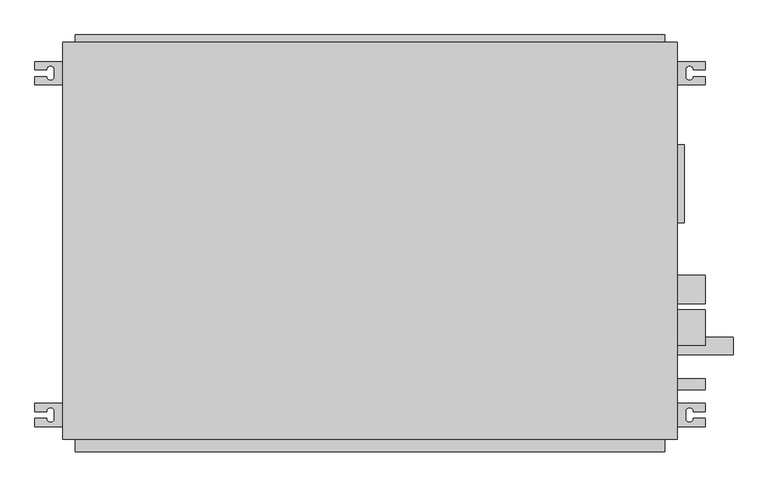
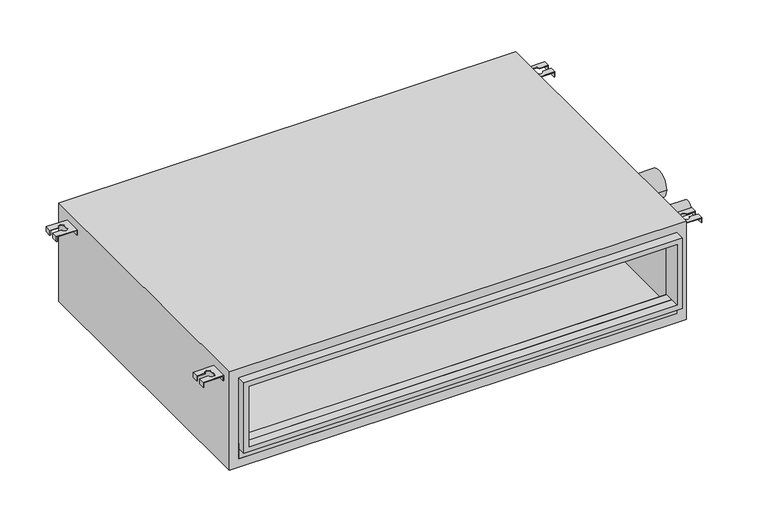
"""IFC4 building model written with IfcOpenShell, lengths in millimetres: proxy geometry, PEFY-P-NMAU-E_Medium_Static_Ducted : PEFY-P30NMAU-E."""

from ifc_helpers import new_model, si_unit, point, frame, frame_2d, origin, place, context, project, spatial, polyline, circle_curve, trimmed, segment, composite_curve, outline, extrude, source, transform, mapped, element, save
from ifc_brep_helpers import plane_surface, revolved_surface, advanced_brep


def mechanical_equipment_d42a0ae8(model_context):
    return source(origin(), model_context, "Body", "SolidModel", [
        advanced_brep(
        [(-610.087243, -231.05, 249.2375), (-610.087243, -246.05, 249.2375), (-589.080993, -246.05, 249.2375), (-575.080993, -246.05, 249.2375), (-575.080993, -258.05, 249.2375), (-589.080993, -258.05, 249.2375), (-610.087243, -258.05, 249.2375), (-610.087243, -273.05, 249.2375), (-560.080993, -273.05, 249.2375), (-560.080993, -231.05, 249.2375), (-610.087243, -231.05, 236.4972162), (-608.499243, -231.05, 236.4972162), (-608.499243, -246.05, 236.4972162), (-610.087243, -246.05, 236.4972162), (-608.499243, -273.05, 236.4972162), (-610.087243, -273.05, 236.4972162), (-610.087243, -258.05, 236.4972162), (-608.499243, -258.05, 236.4972162), (-560.080993, -231.05, 236.4972162), (-560.080993, -273.05, 236.4972162), (-561.668993, -273.05, 236.4972162), (-561.668993, -231.05, 236.4972162), (-608.499243, -246.05, 247.65), (-589.080993, -246.05, 247.65), (-608.499243, -231.05, 247.65), (-561.668993, -231.05, 247.65), (-608.499243, -258.05, 247.65), (-608.499243, -273.05, 247.65), (-589.080993, -258.05, 247.65), (-561.668993, -273.05, 247.65), (-575.080993, -258.05, 247.65), (-575.080993, -246.05, 247.65)],
        [
            (0, 1),
            (1, 2),
            (2, 3, circle_curve(frame((-582.080993, -246.05, 249.2375), z_axis=(0.0, 0.0, -1.0), x_axis=(1.0, 0.0, 0.0)), 7.0)),
            (3, 4),
            (4, 5, circle_curve(frame((-582.080993, -258.05, 249.2375), z_axis=(0.0, 0.0, -1.0), x_axis=(1.0, 0.0, 0.0)), 7.0)),
            (5, 6),
            (6, 7),
            (7, 8),
            (8, 9),
            (9, 0),
            (10, 11),
            (11, 12),
            (12, 13),
            (13, 10),
            (14, 15),
            (15, 16),
            (16, 17),
            (17, 14),
            (18, 19),
            (19, 20),
            (20, 21),
            (21, 18),
            (13, 1),
            (0, 10),
            (12, 22),
            (22, 23),
            (23, 2),
            (11, 24),
            (24, 22),
            (9, 18),
            (21, 25),
            (25, 24),
            (17, 26),
            (26, 27),
            (27, 14),
            (5, 28),
            (28, 26),
            (16, 6),
            (15, 7),
            (27, 29),
            (29, 20),
            (19, 8),
            (29, 25),
            (30, 31),
            (31, 23, circle_curve(frame((-582.080993, -246.05, 247.65), z_axis=(0.0, 0.0, 1.0), x_axis=(1.0, 0.0, 0.0)), 7.0)),
            (28, 30, circle_curve(frame((-582.080993, -258.05, 247.65), z_axis=(0.0, 0.0, 1.0), x_axis=(1.0, 0.0, 0.0)), 7.0)),
            (4, 30),
            (31, 3),
        ],
        [
            plane_surface(frame((-610.087243, -231.05, 249.2375), z_axis=(0.0, 0.0, 1.0), x_axis=(0.0, -1.0, 0.0))),
            plane_surface(frame((-610.087243, -231.05, 236.4972162), z_axis=(0.0, 0.0, -1.0), x_axis=(0.0, 1.0, 0.0))),
            plane_surface(frame((-610.087243, -231.05, 249.2375), z_axis=(-1.0, 0.0, 0.0), x_axis=(0.0, 0.0, -1.0))),
            plane_surface(frame((-610.087243, -246.05, 249.2375), z_axis=(0.0, -1.0, 0.0), x_axis=(0.0, 0.0, -1.0))),
            plane_surface(frame((-608.499243, -246.05, 249.2375), z_axis=(1.0, 0.0, 0.0), x_axis=(0.0, 0.0, -1.0))),
            plane_surface(frame((-608.499243, -231.05, 249.2375), z_axis=(0.0, 1.0, 0.0), x_axis=(0.0, 0.0, -1.0))),
            plane_surface(frame((-608.499243, -273.05, 249.2375), z_axis=(1.0, 0.0, 0.0), x_axis=(0.0, 0.0, -1.0))),
            plane_surface(frame((-608.499243, -258.05, 249.2375), z_axis=(0.0, 1.0, 0.0), x_axis=(0.0, 0.0, -1.0))),
            plane_surface(frame((-610.087243, -258.05, 249.2375), z_axis=(-1.0, 0.0, 0.0), x_axis=(0.0, 0.0, -1.0))),
            plane_surface(frame((-610.087243, -273.05, 249.2375), z_axis=(0.0, -1.0, 0.0), x_axis=(0.0, 0.0, -1.0))),
            plane_surface(frame((-561.668993, -231.05, 249.2375), z_axis=(-1.0, 0.0, 0.0), x_axis=(0.0, 0.0, -1.0))),
            plane_surface(frame((-560.080993, -273.05, 249.2375), z_axis=(1.0, 0.0, 0.0), x_axis=(0.0, 0.0, -1.0))),
            plane_surface(frame((-575.080993, -258.05, 247.65), z_axis=(0.0, 0.0, -1.0), x_axis=(0.0, 1.0, 0.0))),
            revolved_surface(polyline([(-575.080993, -258.05, 247.65), (-575.080993, -258.05, 249.2375)]), (-582.080993, -258.05, 247.65), (0.0, 0.0, -1.0)),
            revolved_surface(polyline([(-575.080993, -246.05, 247.65), (-575.080993, -246.05, 249.2375)]), (-582.080993, -246.05, 247.65), (0.0, 0.0, -1.0)),
            plane_surface(frame((-575.080993, -246.05, 249.2375), z_axis=(-1.0, 0.0, 0.0), x_axis=(0.0, 0.0, -1.0))),
        ],
        [
            (0, [[1, 2, 3, 4, 5, 6, 7, 8, 9, 10]]),
            (1, [[11, 12, 13, 14]]),
            (1, [[15, 16, 17, 18]]),
            (1, [[19, 20, 21, 22]]),
            (2, [[23, -1, 24, -14]]),
            (3, [[-2, -23, -13, 25, 26, 27]]),
            (4, [[-12, 28, 29, -25]]),
            (5, [[-10, 30, -22, 31, 32, -28, -11, -24]]),
            (6, [[-18, 33, 34, 35]]),
            (7, [[-6, 36, 37, -33, -17, 38]]),
            (8, [[39, -7, -38, -16]]),
            (9, [[-8, -39, -15, -35, 40, 41, -20, 42]]),
            (10, [[-21, -41, 43, -31]]),
            (11, [[-30, -9, -42, -19]]),
            (12, [[44, 45, -26, -29, -32, -43, -40, -34, -37, 46]]),
            (13, [[-5, 47, -46, -36]]),
            (14, [[-3, -27, -45, 48]]),
            (15, [[-4, -48, -44, -47]]),
        ],
    ),
        advanced_brep(
        [(590.062757, -231.05, 249.2375), (540.056507, -231.05, 249.2375), (540.056507, -273.05, 249.2375), (590.062757, -273.05, 249.2375), (590.062757, -258.05, 249.2375), (569.056507, -258.05, 249.2375), (555.056507, -258.05, 249.2375), (555.056507, -246.05, 249.2375), (569.056507, -246.05, 249.2375), (590.062757, -246.05, 249.2375), (590.062757, -231.05, 236.4972162), (590.062757, -246.05, 236.4972162), (588.474757, -246.05, 236.4972162), (588.474757, -231.05, 236.4972162), (588.474757, -273.05, 236.4972162), (588.474757, -258.05, 236.4972162), (590.062757, -258.05, 236.4972162), (590.062757, -273.05, 236.4972162), (540.056507, -231.05, 236.4972162), (541.644507, -231.05, 236.4972162), (541.644507, -273.05, 236.4972162), (540.056507, -273.05, 236.4972162), (569.056507, -246.05, 247.65), (588.474757, -246.05, 247.65), (588.474757, -231.05, 247.65), (541.644507, -231.05, 247.65), (588.474757, -273.05, 247.65), (588.474757, -258.05, 247.65), (569.056507, -258.05, 247.65), (541.644507, -273.05, 247.65), (555.056507, -258.05, 247.65), (555.056507, -246.05, 247.65)],
        [
            (0, 1),
            (1, 2),
            (2, 3),
            (3, 4),
            (4, 5),
            (5, 6, circle_curve(frame((562.056507, -258.05, 249.2375), z_axis=(0.0, 0.0, -1.0), x_axis=(-1.0, 0.0, 0.0)), 7.0)),
            (6, 7),
            (7, 8, circle_curve(frame((562.056507, -246.05, 249.2375), z_axis=(0.0, 0.0, -1.0), x_axis=(-1.0, 0.0, 0.0)), 7.0)),
            (8, 9),
            (9, 0),
            (10, 11),
            (11, 12),
            (12, 13),
            (13, 10),
            (14, 15),
            (15, 16),
            (16, 17),
            (17, 14),
            (18, 19),
            (19, 20),
            (20, 21),
            (21, 18),
            (10, 0),
            (9, 11),
            (8, 22),
            (22, 23),
            (23, 12),
            (23, 24),
            (24, 13),
            (24, 25),
            (25, 19),
            (18, 1),
            (14, 26),
            (26, 27),
            (27, 15),
            (4, 16),
            (27, 28),
            (28, 5),
            (3, 17),
            (2, 21),
            (20, 29),
            (29, 26),
            (25, 29),
            (30, 28, circle_curve(frame((562.056507, -258.05, 247.65), z_axis=(0.0, 0.0, 1.0), x_axis=(-1.0, 0.0, 0.0)), 7.0)),
            (22, 31, circle_curve(frame((562.056507, -246.05, 247.65), z_axis=(0.0, 0.0, 1.0), x_axis=(-1.0, 0.0, 0.0)), 7.0)),
            (31, 30),
            (30, 6),
            (7, 31),
        ],
        [
            plane_surface(frame((590.062757, -231.05, 249.2375), z_axis=(0.0, 0.0, 1.0), x_axis=(0.0, -1.0, 0.0))),
            plane_surface(frame((590.062757, -231.05, 236.4972162), z_axis=(0.0, 0.0, -1.0), x_axis=(0.0, 1.0, 0.0))),
            plane_surface(frame((590.062757, -231.05, 249.2375), z_axis=(1.0, 0.0, 0.0), x_axis=(0.0, 0.0, -1.0))),
            plane_surface(frame((590.062757, -246.05, 249.2375), z_axis=(0.0, -1.0, 0.0), x_axis=(0.0, 0.0, -1.0))),
            plane_surface(frame((588.474757, -246.05, 249.2375), z_axis=(-1.0, 0.0, 0.0), x_axis=(0.0, 0.0, -1.0))),
            plane_surface(frame((588.474757, -231.05, 249.2375), z_axis=(0.0, 1.0, 0.0), x_axis=(0.0, 0.0, -1.0))),
            plane_surface(frame((588.474757, -273.05, 249.2375), z_axis=(-1.0, 0.0, 0.0), x_axis=(0.0, 0.0, -1.0))),
            plane_surface(frame((588.474757, -258.05, 249.2375), z_axis=(0.0, 1.0, 0.0), x_axis=(0.0, 0.0, -1.0))),
            plane_surface(frame((590.062757, -258.05, 249.2375), z_axis=(1.0, 0.0, 0.0), x_axis=(0.0, 0.0, -1.0))),
            plane_surface(frame((590.062757, -273.05, 249.2375), z_axis=(0.0, -1.0, 0.0), x_axis=(0.0, 0.0, -1.0))),
            plane_surface(frame((541.644507, -231.05, 249.2375), z_axis=(1.0, 0.0, 0.0), x_axis=(0.0, 0.0, -1.0))),
            plane_surface(frame((540.056507, -273.05, 249.2375), z_axis=(-1.0, 0.0, 0.0), x_axis=(0.0, 0.0, -1.0))),
            plane_surface(frame((555.056507, -258.05, 247.65), z_axis=(0.0, 0.0, -1.0), x_axis=(0.0, 1.0, 0.0))),
            revolved_surface(polyline([(555.056507, -258.05, 247.65), (555.056507, -258.05, 249.2375)]), (562.056507, -258.05, 247.65), (0.0, 0.0, -1.0)),
            revolved_surface(polyline([(555.056507, -246.05, 247.65), (555.056507, -246.05, 249.2375)]), (562.056507, -246.05, 247.65), (0.0, 0.0, -1.0)),
            plane_surface(frame((555.056507, -246.05, 249.2375), z_axis=(1.0, 0.0, 0.0), x_axis=(0.0, 0.0, -1.0))),
        ],
        [
            (0, [[1, 2, 3, 4, 5, 6, 7, 8, 9, 10]]),
            (1, [[11, 12, 13, 14]]),
            (1, [[15, 16, 17, 18]]),
            (1, [[19, 20, 21, 22]]),
            (2, [[-11, 23, -10, 24]]),
            (3, [[25, 26, 27, -12, -24, -9]]),
            (4, [[-27, 28, 29, -13]]),
            (5, [[-23, -14, -29, 30, 31, -19, 32, -1]]),
            (6, [[33, 34, 35, -15]]),
            (7, [[36, -16, -35, 37, 38, -5]]),
            (8, [[-17, -36, -4, 39]]),
            (9, [[40, -21, 41, 42, -33, -18, -39, -3]]),
            (10, [[-31, 43, -41, -20]]),
            (11, [[-22, -40, -2, -32]]),
            (12, [[44, -37, -34, -42, -43, -30, -28, -26, 45, 46]]),
            (13, [[-38, -44, 47, -6]]),
            (14, [[48, -45, -25, -8]]),
            (15, [[-47, -46, -48, -7]]),
        ],
    ),
        advanced_brep(
        [(-610.087243, 339.0, 249.2375), (-560.080993, 339.0, 249.2375), (-560.080993, 381.0, 249.2375), (-610.087243, 381.0, 249.2375), (-610.087243, 366.0, 249.2375), (-589.080993, 366.0, 249.2375), (-575.080993, 366.0, 249.2375), (-575.080993, 354.0, 249.2375), (-589.080993, 354.0, 249.2375), (-610.087243, 354.0, 249.2375), (-610.087243, 339.0, 236.4972162), (-610.087243, 354.0, 236.4972162), (-608.499243, 354.0, 236.4972162), (-608.499243, 339.0, 236.4972162), (-608.499243, 381.0, 236.4972162), (-608.499243, 366.0, 236.4972162), (-610.087243, 366.0, 236.4972162), (-610.087243, 381.0, 236.4972162), (-560.080993, 339.0, 236.4972162), (-561.668993, 339.0, 236.4972162), (-561.668993, 381.0, 236.4972162), (-560.080993, 381.0, 236.4972162), (-589.080993, 354.0, 247.65), (-608.499243, 354.0, 247.65), (-608.499243, 339.0, 247.65), (-561.668993, 339.0, 247.65), (-608.499243, 381.0, 247.65), (-608.499243, 366.0, 247.65), (-589.080993, 366.0, 247.65), (-561.668993, 381.0, 247.65), (-575.080993, 366.0, 247.65), (-575.080993, 354.0, 247.65)],
        [
            (0, 1),
            (1, 2),
            (2, 3),
            (3, 4),
            (4, 5),
            (5, 6, circle_curve(frame((-582.080993, 366.0, 249.2375), z_axis=(0.0, 0.0, -1.0), x_axis=(1.0, 0.0, 0.0)), 7.0)),
            (6, 7),
            (7, 8, circle_curve(frame((-582.080993, 354.0, 249.2375), z_axis=(0.0, 0.0, -1.0), x_axis=(1.0, 0.0, 0.0)), 7.0)),
            (8, 9),
            (9, 0),
            (10, 11),
            (11, 12),
            (12, 13),
            (13, 10),
            (14, 15),
            (15, 16),
            (16, 17),
            (17, 14),
            (18, 19),
            (19, 20),
            (20, 21),
            (21, 18),
            (10, 0),
            (9, 11),
            (8, 22),
            (22, 23),
            (23, 12),
            (23, 24),
            (24, 13),
            (24, 25),
            (25, 19),
            (18, 1),
            (14, 26),
            (26, 27),
            (27, 15),
            (4, 16),
            (27, 28),
            (28, 5),
            (3, 17),
            (2, 21),
            (20, 29),
            (29, 26),
            (25, 29),
            (30, 28, circle_curve(frame((-582.080993, 366.0, 247.65), z_axis=(0.0, 0.0, 1.0), x_axis=(1.0, 0.0, 0.0)), 7.0)),
            (22, 31, circle_curve(frame((-582.080993, 354.0, 247.65), z_axis=(0.0, 0.0, 1.0), x_axis=(1.0, 0.0, 0.0)), 7.0)),
            (31, 30),
            (30, 6),
            (7, 31),
        ],
        [
            plane_surface(frame((-610.087243, 339.0, 249.2375), z_axis=(0.0, 0.0, 1.0), x_axis=(0.0, 1.0, 0.0))),
            plane_surface(frame((-610.087243, 339.0, 236.4972162), z_axis=(0.0, 0.0, -1.0), x_axis=(0.0, -1.0, 0.0))),
            plane_surface(frame((-610.087243, 339.0, 249.2375), z_axis=(-1.0, 0.0, 0.0), x_axis=(0.0, 0.0, -1.0))),
            plane_surface(frame((-610.087243, 354.0, 249.2375), z_axis=(0.0, 1.0, 0.0), x_axis=(0.0, 0.0, -1.0))),
            plane_surface(frame((-608.499243, 354.0, 249.2375), z_axis=(1.0, 0.0, 0.0), x_axis=(0.0, 0.0, -1.0))),
            plane_surface(frame((-608.499243, 339.0, 249.2375), z_axis=(0.0, -1.0, 0.0), x_axis=(0.0, 0.0, -1.0))),
            plane_surface(frame((-608.499243, 381.0, 249.2375), z_axis=(1.0, 0.0, 0.0), x_axis=(0.0, 0.0, -1.0))),
            plane_surface(frame((-608.499243, 366.0, 249.2375), z_axis=(0.0, -1.0, 0.0), x_axis=(0.0, 0.0, -1.0))),
            plane_surface(frame((-610.087243, 366.0, 249.2375), z_axis=(-1.0, 0.0, 0.0), x_axis=(0.0, 0.0, -1.0))),
            plane_surface(frame((-610.087243, 381.0, 249.2375), z_axis=(0.0, 1.0, 0.0), x_axis=(0.0, 0.0, -1.0))),
            plane_surface(frame((-561.668993, 339.0, 249.2375), z_axis=(-1.0, 0.0, 0.0), x_axis=(0.0, 0.0, -1.0))),
            plane_surface(frame((-560.080993, 381.0, 249.2375), z_axis=(1.0, 0.0, 0.0), x_axis=(0.0, 0.0, -1.0))),
            plane_surface(frame((-575.080993, 366.0, 247.65), z_axis=(0.0, 0.0, -1.0), x_axis=(0.0, -1.0, 0.0))),
            revolved_surface(polyline([(-575.080993, 366.0, 247.65), (-575.080993, 366.0, 249.2375)]), (-582.080993, 366.0, 247.65), (0.0, 0.0, -1.0)),
            revolved_surface(polyline([(-575.080993, 354.0, 247.65), (-575.080993, 354.0, 249.2375)]), (-582.080993, 354.0, 247.65), (0.0, 0.0, -1.0)),
            plane_surface(frame((-575.080993, 354.0, 249.2375), z_axis=(-1.0, 0.0, 0.0), x_axis=(0.0, 0.0, -1.0))),
        ],
        [
            (0, [[1, 2, 3, 4, 5, 6, 7, 8, 9, 10]]),
            (1, [[11, 12, 13, 14]]),
            (1, [[15, 16, 17, 18]]),
            (1, [[19, 20, 21, 22]]),
            (2, [[-11, 23, -10, 24]]),
            (3, [[25, 26, 27, -12, -24, -9]]),
            (4, [[-27, 28, 29, -13]]),
            (5, [[-23, -14, -29, 30, 31, -19, 32, -1]]),
            (6, [[33, 34, 35, -15]]),
            (7, [[36, -16, -35, 37, 38, -5]]),
            (8, [[-17, -36, -4, 39]]),
            (9, [[40, -21, 41, 42, -33, -18, -39, -3]]),
            (10, [[-31, 43, -41, -20]]),
            (11, [[-22, -40, -2, -32]]),
            (12, [[44, -37, -34, -42, -43, -30, -28, -26, 45, 46]]),
            (13, [[-38, -44, 47, -6]]),
            (14, [[48, -45, -25, -8]]),
            (15, [[-47, -46, -48, -7]]),
        ],
    ),
        advanced_brep(
        [(590.062757, 339.0, 249.2375), (590.062757, 354.0, 249.2375), (569.056507, 354.0, 249.2375), (555.056507, 354.0, 249.2375), (555.056507, 366.0, 249.2375), (569.056507, 366.0, 249.2375), (590.062757, 366.0, 249.2375), (590.062757, 381.0, 249.2375), (540.056507, 381.0, 249.2375), (540.056507, 339.0, 249.2375), (590.062757, 339.0, 236.4972162), (588.474757, 339.0, 236.4972162), (588.474757, 354.0, 236.4972162), (590.062757, 354.0, 236.4972162), (588.474757, 381.0, 236.4972162), (590.062757, 381.0, 236.4972162), (590.062757, 366.0, 236.4972162), (588.474757, 366.0, 236.4972162), (540.056507, 339.0, 236.4972162), (540.056507, 381.0, 236.4972162), (541.644507, 381.0, 236.4972162), (541.644507, 339.0, 236.4972162), (588.474757, 354.0, 247.65), (569.056507, 354.0, 247.65), (588.474757, 339.0, 247.65), (541.644507, 339.0, 247.65), (588.474757, 366.0, 247.65), (588.474757, 381.0, 247.65), (569.056507, 366.0, 247.65), (541.644507, 381.0, 247.65), (555.056507, 366.0, 247.65), (555.056507, 354.0, 247.65)],
        [
            (0, 1),
            (1, 2),
            (2, 3, circle_curve(frame((562.056507, 354.0, 249.2375), z_axis=(0.0, 0.0, -1.0), x_axis=(-1.0, 0.0, 0.0)), 7.0)),
            (3, 4),
            (4, 5, circle_curve(frame((562.056507, 366.0, 249.2375), z_axis=(0.0, 0.0, -1.0), x_axis=(-1.0, 0.0, 0.0)), 7.0)),
            (5, 6),
            (6, 7),
            (7, 8),
            (8, 9),
            (9, 0),
            (10, 11),
            (11, 12),
            (12, 13),
            (13, 10),
            (14, 15),
            (15, 16),
            (16, 17),
            (17, 14),
            (18, 19),
            (19, 20),
            (20, 21),
            (21, 18),
            (13, 1),
            (0, 10),
            (12, 22),
            (22, 23),
            (23, 2),
            (11, 24),
            (24, 22),
            (9, 18),
            (21, 25),
            (25, 24),
            (17, 26),
            (26, 27),
            (27, 14),
            (5, 28),
            (28, 26),
            (16, 6),
            (15, 7),
            (27, 29),
            (29, 20),
            (19, 8),
            (29, 25),
            (30, 31),
            (31, 23, circle_curve(frame((562.056507, 354.0, 247.65), z_axis=(0.0, 0.0, 1.0), x_axis=(-1.0, 0.0, 0.0)), 7.0)),
            (28, 30, circle_curve(frame((562.056507, 366.0, 247.65), z_axis=(0.0, 0.0, 1.0), x_axis=(-1.0, 0.0, 0.0)), 7.0)),
            (4, 30),
            (31, 3),
        ],
        [
            plane_surface(frame((590.062757, 339.0, 249.2375), z_axis=(0.0, 0.0, 1.0), x_axis=(0.0, 1.0, 0.0))),
            plane_surface(frame((590.062757, 339.0, 236.4972162), z_axis=(0.0, 0.0, -1.0), x_axis=(0.0, -1.0, 0.0))),
            plane_surface(frame((590.062757, 339.0, 249.2375), z_axis=(1.0, 0.0, 0.0), x_axis=(0.0, 0.0, -1.0))),
            plane_surface(frame((590.062757, 354.0, 249.2375), z_axis=(0.0, 1.0, 0.0), x_axis=(0.0, 0.0, -1.0))),
            plane_surface(frame((588.474757, 354.0, 249.2375), z_axis=(-1.0, 0.0, 0.0), x_axis=(0.0, 0.0, -1.0))),
            plane_surface(frame((588.474757, 339.0, 249.2375), z_axis=(0.0, -1.0, 0.0), x_axis=(0.0, 0.0, -1.0))),
            plane_surface(frame((588.474757, 381.0, 249.2375), z_axis=(-1.0, 0.0, 0.0), x_axis=(0.0, 0.0, -1.0))),
            plane_surface(frame((588.474757, 366.0, 249.2375), z_axis=(0.0, -1.0, 0.0), x_axis=(0.0, 0.0, -1.0))),
            plane_surface(frame((590.062757, 366.0, 249.2375), z_axis=(1.0, 0.0, 0.0), x_axis=(0.0, 0.0, -1.0))),
            plane_surface(frame((590.062757, 381.0, 249.2375), z_axis=(0.0, 1.0, 0.0), x_axis=(0.0, 0.0, -1.0))),
            plane_surface(frame((541.644507, 339.0, 249.2375), z_axis=(1.0, 0.0, 0.0), x_axis=(0.0, 0.0, -1.0))),
            plane_surface(frame((540.056507, 381.0, 249.2375), z_axis=(-1.0, 0.0, 0.0), x_axis=(0.0, 0.0, -1.0))),
            plane_surface(frame((555.056507, 366.0, 247.65), z_axis=(0.0, 0.0, -1.0), x_axis=(0.0, -1.0, 0.0))),
            revolved_surface(polyline([(555.056507, 366.0, 247.65), (555.056507, 366.0, 249.2375)]), (562.056507, 366.0, 247.65), (0.0, 0.0, -1.0)),
            revolved_surface(polyline([(555.056507, 354.0, 247.65), (555.056507, 354.0, 249.2375)]), (562.056507, 354.0, 247.65), (0.0, 0.0, -1.0)),
            plane_surface(frame((555.056507, 354.0, 249.2375), z_axis=(1.0, 0.0, 0.0), x_axis=(0.0, 0.0, -1.0))),
        ],
        [
            (0, [[1, 2, 3, 4, 5, 6, 7, 8, 9, 10]]),
            (1, [[11, 12, 13, 14]]),
            (1, [[15, 16, 17, 18]]),
            (1, [[19, 20, 21, 22]]),
            (2, [[23, -1, 24, -14]]),
            (3, [[-2, -23, -13, 25, 26, 27]]),
            (4, [[-12, 28, 29, -25]]),
            (5, [[-10, 30, -22, 31, 32, -28, -11, -24]]),
            (6, [[-18, 33, 34, 35]]),
            (7, [[-6, 36, 37, -33, -17, 38]]),
            (8, [[39, -7, -38, -16]]),
            (9, [[-8, -39, -15, -35, 40, 41, -20, 42]]),
            (10, [[-21, -41, 43, -31]]),
            (11, [[-30, -9, -42, -19]]),
            (12, [[44, 45, -26, -29, -32, -43, -40, -34, -37, 46]]),
            (13, [[-5, 47, -46, -36]]),
            (14, [[-3, -27, -45, 48]]),
            (15, [[-4, -48, -44, -47]]),
        ],
    ),
        extrude(outline(polyline([(517.831507, -295.275), (-537.855993, -295.275), (-537.855993, -273.05), (517.831507, -273.05), (517.831507, -295.275)])), frame((0.0, 0.0, 42.8625), z_axis=(0.0, 0.0, 1.0), x_axis=(1.0, 0.0, 0.0)), (0.0, 0.0, 1.0), 39.6875),
        extrude(outline(polyline([(249.2375, 517.831507), (249.2375, -537.855993), (69.85, -537.855993), (69.85, 517.831507), (249.2375, 517.831507)]), holes=[polyline([(82.55, 505.131507), (82.55, -525.155993), (236.5375, -525.155993), (236.5375, 505.131507), (82.55, 505.131507)])]), frame((0.0, -317.5, 0.0), z_axis=(0.0, 1.0, 0.0), x_axis=(0.0, 0.0, 1.0)), (0.0, 0.0, 1.0), 44.45),
        extrude(outline(polyline([(517.831507, 415.925), (-537.855993, 415.925), (-537.855993, 428.625), (517.831507, 428.625), (517.831507, 415.925)])), frame((0.0, 0.0, 42.8625), z_axis=(0.0, 0.0, 1.0), x_axis=(1.0, 0.0, 0.0)), (0.0, 0.0, 1.0), 206.375),
        extrude(outline(polyline([(271.4625, 540.056507), (271.4625, -560.080993), (20.6375, -560.080993), (20.6375, 540.056507), (271.4625, 540.056507)]), holes=[polyline([(42.8625, -537.855993), (249.2375, -537.855993), (249.2375, 517.831507), (42.8625, 517.831507), (42.8625, -537.855993)])]), frame((0.0, -295.275, 0.0), z_axis=(0.0, 1.0, 0.0), x_axis=(0.0, 0.0, 1.0)), (0.0, 0.0, 1.0), 711.2),
        extrude(outline(composite_curve([segment(trimmed(circle_curve(frame_2d((-26.9875, 109.5375)), 25.4), [point((-1.5875, 109.5375))], [point((-52.3875, 109.5375))], False, "CARTESIAN"), True, "CONTINUOUS"), segment(trimmed(circle_curve(frame_2d((-26.9875, 109.5375)), 25.4), [point((-52.3875, 109.5375))], [point((-1.5875, 109.5375))], False, "CARTESIAN"), True, "CONTINUOUS")], self_intersect=False)), frame((540.056507, 0.0, 0.0), z_axis=(1.0, 0.0, 0.0), x_axis=(0.0, 1.0, 0.0)), (0.0, 0.0, 1.0), 50.00625),
        extrude(outline(composite_curve([segment(trimmed(circle_curve(frame_2d((-128.5875, 171.45)), 15.875), [point((-112.7125, 171.45))], [point((-144.4625, 171.45))], False, "CARTESIAN"), True, "CONTINUOUS"), segment(trimmed(circle_curve(frame_2d((-128.5875, 171.45)), 15.875), [point((-144.4625, 171.45))], [point((-112.7125, 171.45))], False, "CARTESIAN"), True, "CONTINUOUS")], self_intersect=False)), frame((540.056507, 0.0, 0.0), z_axis=(1.0, 0.0, 0.0), x_axis=(0.0, 1.0, 0.0)), (0.0, 0.0, 1.0), 100.0125),
        extrude(outline(composite_curve([segment(trimmed(circle_curve(frame_2d((-95.25, 230.1875)), 31.75), [point((-63.5, 230.1875))], [point((-127.0, 230.1875))], False, "CARTESIAN"), True, "CONTINUOUS"), segment(trimmed(circle_curve(frame_2d((-95.25, 230.1875)), 31.75), [point((-127.0, 230.1875))], [point((-63.5, 230.1875))], False, "CARTESIAN"), True, "CONTINUOUS")], self_intersect=False)), frame((540.056507, 0.0, 0.0), z_axis=(1.0, 0.0, 0.0), x_axis=(0.0, 1.0, 0.0)), (0.0, 0.0, 1.0), 50.00625),
        extrude(outline(composite_curve([segment(trimmed(circle_curve(frame_2d((-196.85, 104.775)), 9.525), [point((-187.325, 104.775))], [point((-206.375, 104.775))], False, "CARTESIAN"), True, "CONTINUOUS"), segment(trimmed(circle_curve(frame_2d((-196.85, 104.775)), 9.525), [point((-206.375, 104.775))], [point((-187.325, 104.775))], False, "CARTESIAN"), True, "CONTINUOUS")], self_intersect=False)), frame((540.056507, 0.0, 0.0), z_axis=(1.0, 0.0, 0.0), x_axis=(0.0, 1.0, 0.0)), (0.0, 0.0, 1.0), 50.00625),
        extrude(outline(polyline([(552.756507, 231.84375), (552.756507, 92.14375), (540.056507, 92.14375), (540.056507, 231.84375), (552.756507, 231.84375)])), frame((0.0, 0.0, 42.8625), z_axis=(0.0, 0.0, 1.0), x_axis=(1.0, 0.0, 0.0)), (0.0, 0.0, 1.0), 187.325),
    ])


if __name__ == "__main__":
    model = new_model("IFC4")
    model_context = context("Model", 3, world=origin())
    ifc_project = project(units=[si_unit("LENGTHUNIT", "METRE", prefix="MILLI")], contexts=[model_context])
    site = spatial("IfcSite", under=ifc_project)
    building = spatial("IfcBuilding", under=site)
    placement = place(None, origin())
    mechanical_equipment_shape = mechanical_equipment_d42a0ae8(model_context)
    element("IfcBuildingElementProxy", 1, Name="PEFY-P-NMAU-E_Medium_Static_Ducted : PEFY-P30NMAU-E", ObjectType="PEFY-P-NMAU-E_Medium_Static_Ducted : PEFY-P30NMAU-E", at=placement, inside=building, context=model_context, shape_type="MappedRepresentation", body=[
        mapped(mechanical_equipment_shape, transform((0.0, 0.0, 0.0), x_axis=(1.0, 0.0, 0.0), y_axis=(0.0, 1.0, 0.0), z_axis=(0.0, 0.0, 1.0))),
    ])
    save(model, "model.ifc")

# Revit data of these elements
# Type "PEFY-P-NMAU-E_Medium_Static_Ducted : PEFY-P30NMAU-E"
#   Wiring (Min.size of wire) = "1/8"
#   Wiring (Amperage of wire breaker) = "15 A"
#   Voltage Options = "208/230 VAC"
#   Unit Weight (LBS) = "71"
#   Temperature set range Remote controller Heating = "63 to 83 F"
#   Temperature set range Remote controller Cooling = "67 to 86 F"
#   Subcategory = "HVAC"
#   Specification URL = ""
#   Sound Pressure Levels (dB(A)) = "26,28,29"
#   SmartBIM Object Created By = "Reed Construction Data"
#   Single Phase = "X"
#   Refrigerant control device = "LEV"
#   Protection devices = "Fuse"
#   Power input Heating = "0.12 kW"
#   Power input Cooling = "0.14 kW"
#   Moter Type = "DC blushless motor"
#   Moter Output = "0.085 kW"
#   Model = "PEFY-P30NMAU-E"
#   Manufacturer URL = ""
#   Manufacturer = "Mitsubishi Electric"
#   Insulation material = "EPS, Polyethylene foam, Urethane foam"
#   Installation URL = ""
#   Heating Capacity (kcal/h) = "7,600"
#   Heating Capacity (kW) = "8.8"
#   Heat exchanger = "Cross fin(Aluminium fin and copper tube)"
#   Frequency = "60 Hz"
#   Fan Type x Quantity = "Sirocco fan x 1"
#   E.S.P(mmH2O) = "3.6,5.1,7.1,10.2,15.3"
#   E.S.P(Pa) = "35,50,70,100,150"
#   E.S.P(In. W.G.) = "0.14,0.20,0.28,0.40,0.60"
#   Driving mechanism = "Direct-driven by motor"
#   Current Heating = "1.07 A"
#   Current Cooling = "1.18 A"
#   Cooling Capacity (kcal/h) = "6,800"
#   Cooling Capacity (kW) = "7.9"
#   Connectable outdoor unit = "R410A,R22 CITY MULTI"
#   Assembly Code = "D3050200"
#   Airflow rate(Low-Mid-High) (m3/min) = "6.0,7.5,8.5"
#   Airflow rate(Low-Mid-High) (cfm) = "212,265,300"
#   Airflow rate(Low-Mid-High) (L/s) = "100,125,142"
#   Air Filter = "PP Honeycomb fabric"
#   95 CSI = "15760"
#   04 CSI = "23 82 19"
#   Width = 1100.138 mm
#   Voltage = 0 V
#   Unit Supply Airflow [instance default] = 0 CFM
#   Unit Return Airflow [instance default] = 0 CFM
#   SmartBIM Object Version = 3
#   Refrigerant Pipe Liquid = 9.525 mm
#   Refrigerant Pipe Gas = 15.875 mm
#   Refirigerant Pipe diameter (Liquid) = 9.525 mm
#   Refirigerant Pipe diameter (Gas) = 15.875 mm
#   Phase = 0
#   Nominal Heating Capacity = 34000.0 Btu/h
#   Nominal Cooling Capacity = 30000.0 Btu/h
#   Minimum Circuit Current = 2.5 A
#   Maximum Overcurrent Protection = 15 A
#   Hertz = 0
#   Height = 250.825 mm
#   Drain piping diameter = 31.75 mm
#   Drain Pump = 25.4 mm
#   Depth = 733.425 mm
#   Default Elevation = 1219.2 mm
#   Back Air Inlet Width = 1055.688 mm
#   Back Air Inlet Height = 206.375 mm
#   Apparent Load = 0 VA
#   Air Outlet Width = 1055.688 mm
#   Air Outlet Height = 179.388 mm
#   Sound Pressure Levels @ Mid Airflow (dBA) = 34
#   Sound Pressure Levels @ Low Airflow (dBA) = 30
#   Sound Pressure Levels @ High Airflow (dBA) = 38
#   Number of Poles = 1
#   Unit = Metal - Steel Satin
#   Load Classification = Other
#   Back Air Inlet = Grille
# Element 1 (IfcBuildingElementProxy, "PEFY-P-NMAU-E_Medium_Static_Ducted : PEFY-P30NMAU-E")
#   Unit Supply Airflow = 750 CFM
#   Unit Return Airflow = 750 CFM
#   Materials on its faces: "Metal - Steel Satin", "Grille"
# Materials
#   "Metal - Steel Satin": class "Metal", colour RGB 189 187 185, transparency 0
#   "Grille": class "Miscellaneous", colour RGB 0 0 0, transparency 0
